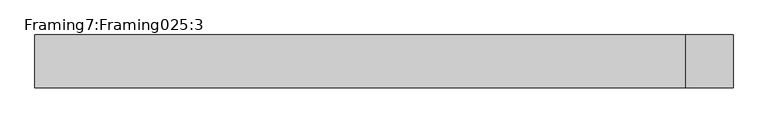
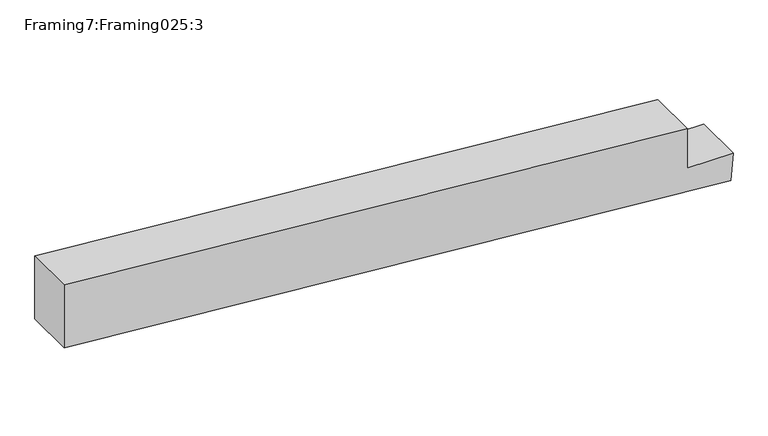
"""IFC4 building model written with IfcOpenShell, lengths in millimetres: proxy geometry, Framing7:Framing025:3 : Framing7:Framing025:286338."""

from ifc_helpers import new_model, si_unit, frame, origin, place, context, project, spatial, polyline, outline, extrude, source, transform, mapped, element, save


def framing7_framing025_3_f3505e93(model_context):
    return source(origin(), model_context, "Body", "SweptSolid", [
        extrude(outline(polyline([(109380.3725016, 15155.7938045), (109465.6286206, 15162.9505222), (109465.6286206, 15023.9855685), (109592.3369486, 15023.9855685), (109750.130283, 13144.2345798), (109549.2303128, 13144.2345798), (109380.3725016, 15155.7938045)])), frame((0.0, -14445.349577, 0.0), z_axis=(0.0, 1.0, 0.0), x_axis=(0.0, 0.0, 1.0)), (0.0, 0.0, 1.0), 152.4),
    ])


if __name__ == "__main__":
    model = new_model("IFC4")
    model_context = context("Model", 3, world=origin())
    ifc_project = project(units=[si_unit("LENGTHUNIT", "METRE", prefix="MILLI")], contexts=[model_context])
    site = spatial("IfcSite", under=ifc_project)
    building = spatial("IfcBuilding", under=site)
    placement = place(None, origin())
    framing7_framing025_3_shape = framing7_framing025_3_f3505e93(model_context)
    element("IfcBuildingElementProxy", 1, Name="Framing7:Framing025:3 : Framing7:Framing025:286338", ObjectType="Framing7:Framing025:3 : Framing7:Framing025:286338", at=placement, inside=building, context=model_context, shape_type="MappedRepresentation", body=[
        mapped(framing7_framing025_3_shape, transform((0.0, 0.0, 0.0), x_axis=(1.0, 0.0, 0.0), y_axis=(0.0, 1.0, 0.0), z_axis=(0.0, 0.0, 1.0))),
    ])
    save(model, "model.ifc")

# Revit data of these elements
# Type "Framing7:Framing025:3 : Framing7:Framing025:286338"
#   NameOverride = "Framing7:Framing025:286338"
#   ObjectTypeOverride = "Framing7:Framing025"
#   Reference = "Framing025"
#   Category = "Generic Models"
#   Tag = "286338"
# Element 1 (IfcBuildingElementProxy, "Framing7:Framing025:3 : Framing7:Framing025:286338")
#   Materials on its faces: "WOOD FRAMING (SEE STRUCT DWGS)"
# Materials
#   "WOOD FRAMING (SEE STRUCT DWGS)": class "Unassigned", colour RGB 224 188 168, transparency 0, Cost = 0
